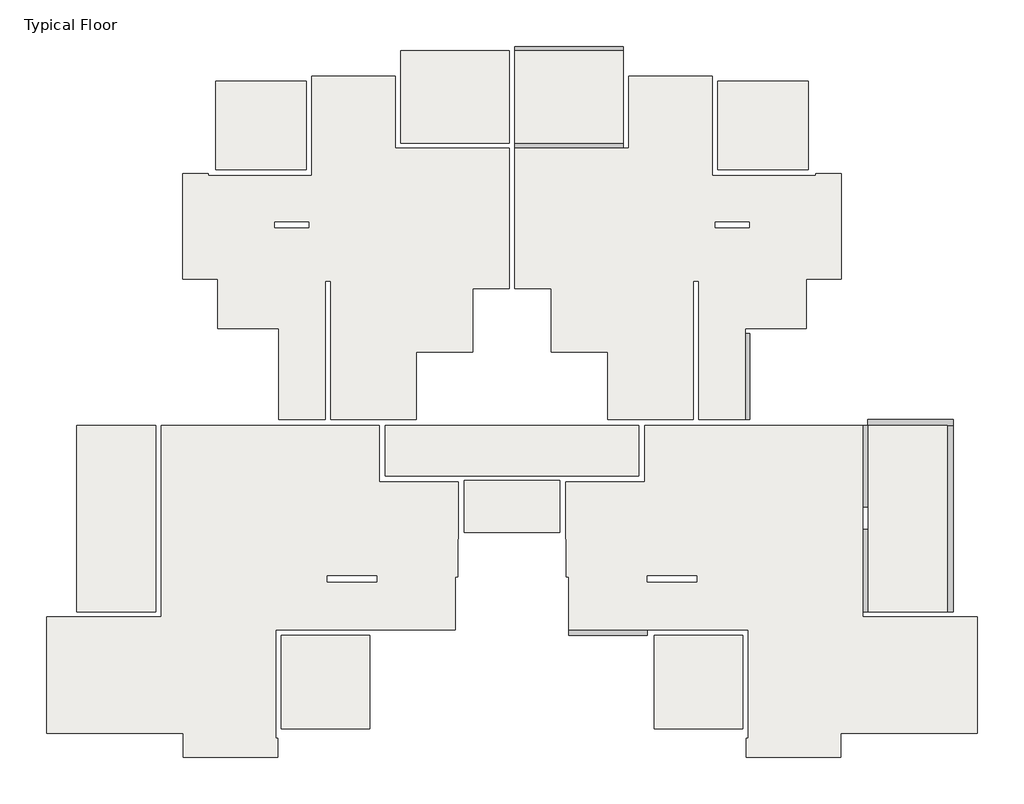
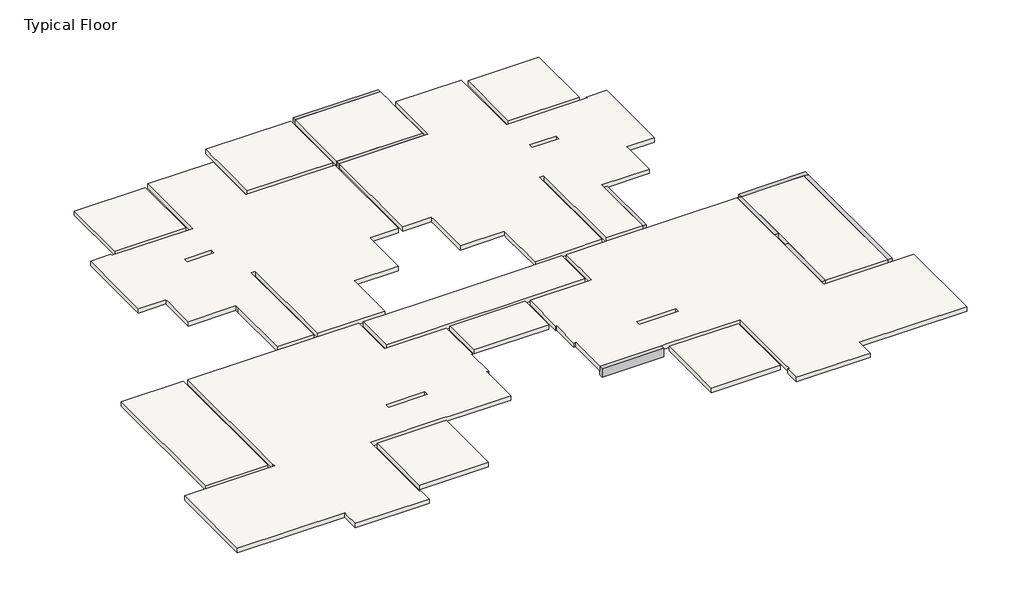
# One storey: 14 slabs, 8 beams.
"""IFC4 building model written with IfcOpenShell, lengths in millimetres."""

from ifc_helpers import new_model, si_unit, frame, origin, place, context, project, spatial, polyline, outline, extrude, faceted_brep, element, save

model = new_model("IFC4")

# Units and contexts
model_context = context("Model", 3, world=origin())
ifc_project = project(units=[si_unit("LENGTHUNIT", "METRE", prefix="MILLI")], contexts=[model_context])

# Site, building, storey
site = spatial("IfcSite", under=ifc_project)
building = spatial("IfcBuilding", under=site)
storey = spatial("IfcBuildingStorey", under=building, Name="Typical Floor", Elevation=2970.0)

# Beams
placement = place(None, origin())
element("IfcBeam", 1, ObjectType="Concrete Rectengular Beam : 15/40", at=placement, inside=storey, context=model_context, shape_type="Brep", body=[
    faceted_brep([(9242.3116422, 3105.4959573, 2970.0), (9092.3116422, 3105.4959573, 2970.0), (9092.3116422, 53.6346435, 2970.0), (9242.3116422, 53.6346435, 2970.0), (9242.3116422, 3105.4959573, 2570.0), (9242.3116422, 53.6346435, 2570.0), (9092.3116422, 3105.4959573, 2570.0), (9092.3116422, 53.6346435, 2570.0), (9092.3116422, 3105.4959573, 2760.0), (9092.3116422, 53.6346435, 2760.0)], [[[0, 1, 2, 3]], [[4, 0, 3, 5]], [[6, 4, 5, 7]], [[2, 1, 8, 6, 7, 9]], [[1, 0, 4, 6, 8]], [[3, 2, 9, 7, 5]]]),
])
element("IfcBeam", 2, ObjectType="Concrete Rectengular Beam : 15/40", at=placement, inside=storey, context=model_context, shape_type="Brep", body=[
    faceted_brep([(4769.8298903, 13127.6127456, 2970.0), (4769.8298903, 13277.6127456, 2970.0), (922.5306203, 13277.6127456, 2970.0), (922.5306203, 13127.6127456, 2970.0), (4769.8298903, 13127.6127456, 2570.0), (4769.8298903, 13127.6127456, 2760.0), (922.5306203, 13127.6127456, 2760.0), (922.5306203, 13127.6127456, 2570.0), (4769.8298903, 13277.6127456, 2570.0), (922.5306203, 13277.6127456, 2570.0)], [[[0, 1, 2, 3]], [[4, 5, 0, 3, 6, 7]], [[8, 4, 7, 9]], [[1, 8, 9, 2]], [[1, 0, 5, 4, 8]], [[3, 2, 9, 7, 6]]]),
])
element("IfcBeam", 3, ObjectType="Concrete Rectengular Beam : 18/40", at=placement, inside=storey, context=model_context, shape_type="Brep", body=[
    faceted_brep([(922.5306203, 9859.0725997, 2970.0), (922.5306203, 9679.0725997, 2970.0), (4769.8298903, 9679.0725997, 2970.0), (4769.8298903, 9859.0725997, 2970.0), (922.5306203, 9679.0725997, 2760.0), (922.5306203, 9679.0725997, 2570.0), (4769.8298903, 9679.0725997, 2570.0), (922.5306203, 9859.0725997, 2570.0), (4769.8298903, 9859.0725997, 2570.0), (922.5306203, 9859.0725997, 2760.0), (4769.8298903, 9859.0725997, 2760.0)], [[[0, 1, 2, 3]], [[1, 4, 5, 6, 2]], [[5, 7, 8, 6]], [[7, 9, 0, 3, 10, 8]], [[1, 0, 9, 7, 5, 4]], [[3, 2, 6, 8, 10]]]),
])
element("IfcBeam", 4, ObjectType="Concrete Rectengular Beam : 20/40", at=placement, inside=storey, context=model_context, shape_type="Brep", body=[
    faceted_brep([(16442.8225911, -146.3653565, 2970.0), (16442.8225911, 53.6346435, 2970.0), (13417.2386495, 53.6346435, 2970.0), (13417.2386495, -146.3653565, 2970.0), (13440.1948538, -146.3653565, 2970.0), (16242.8225911, -146.3653565, 2970.0), (16442.8225911, 53.6346435, 2570.0), (13417.2386495, 53.6346435, 2570.0), (16442.8225911, -146.3653565, 2570.0), (16242.8225911, -146.3653565, 2570.0), (13440.1948538, -146.3653565, 2570.0), (13417.2386495, -146.3653565, 2570.0)], [[[0, 1, 2, 3, 4, 5]], [[1, 6, 7, 2]], [[6, 8, 9, 10, 11, 7]], [[8, 0, 5, 4, 3, 11, 10, 9]], [[3, 2, 7, 11]], [[1, 0, 8, 6]]]),
])
element("IfcBeam", 5, ObjectType="Concrete Rectengular Beam : 20/40", at=placement, inside=storey, context=model_context, shape_type="Brep", body=[
    faceted_brep([(16242.8225911, -6750.8420555, 2970.0), (16442.8225911, -6750.8420555, 2970.0), (16442.8225911, -146.3653565, 2970.0), (16242.8225911, -146.3653565, 2970.0), (16442.8225911, -6750.8420555, 2570.0), (16442.8225911, -146.3653565, 2570.0), (16242.8225911, -6750.8420555, 2570.0), (16242.8225911, -146.3653565, 2570.0), (16242.8225911, -6750.8420555, 2760.0), (16242.8225911, -146.3653565, 2760.0)], [[[0, 1, 2, 3]], [[1, 4, 5, 2]], [[4, 6, 7, 5]], [[6, 8, 0, 3, 9, 7]], [[1, 0, 8, 6, 4]], [[3, 2, 5, 7, 9]]]),
])
element("IfcBeam", 6, ObjectType="Concrete Rectengular Beam : 20/40", at=placement, inside=storey, context=model_context, shape_type="Brep", body=[
    faceted_brep([(13240.1948538, -3042.8252106, 2970.0), (13440.1948538, -3042.8252106, 2970.0), (13440.1948538, -146.3653565, 2970.0), (13417.2386495, -146.3653565, 2970.0), (13240.1948538, -146.3653565, 2970.0), (13440.1948538, -3042.8252106, 2570.0), (13440.1948538, -146.3653565, 2570.0), (13440.1948538, -146.3653565, 2760.0), (13240.1948538, -3042.8252106, 2570.0), (13240.1948538, -146.3653565, 2570.0), (13417.2386495, -146.3653565, 2570.0), (13240.1948538, -146.3653565, 2760.0), (13240.1948538, -3042.8252106, 2760.0)], [[[0, 1, 2, 3, 4]], [[1, 5, 6, 7, 2]], [[5, 8, 9, 10, 6]], [[0, 4, 11, 9, 8, 12]], [[1, 0, 12, 8, 5]], [[2, 7, 6, 10, 9, 11, 4, 3]]]),
])
element("IfcBeam", 7, ObjectType="Concrete Rectengular Beam : 20/40", at=placement, inside=storey, context=model_context, shape_type="Brep", body=[
    faceted_brep([(13440.1948538, -3842.8252106, 2970.0), (13240.1948538, -3842.8252106, 2970.0), (13240.1948538, -6750.8420555, 2970.0), (13440.1948538, -6750.8420555, 2970.0), (13440.1948538, -3842.8252106, 2570.0), (13440.1948538, -6750.8420555, 2760.0), (13440.1948538, -6750.8420555, 2570.0), (13240.1948538, -3842.8252106, 2570.0), (13240.1948538, -6750.8420555, 2570.0), (13240.1948538, -3842.8252106, 2760.0), (13240.1948538, -6750.8420555, 2760.0)], [[[0, 1, 2, 3]], [[4, 0, 3, 5, 6]], [[7, 4, 6, 8]], [[2, 1, 9, 7, 8, 10]], [[1, 0, 4, 7, 9]], [[3, 2, 10, 8, 6, 5]]]),
])
element("IfcBeam", 8, ObjectType="Concrete Rectengular Beam : 20/40", at=placement, inside=storey, context=model_context, shape_type="Brep", body=[
    faceted_brep([(5618.7842881, -7595.8420555, 2970.0), (5618.7842881, -7395.8420555, 2970.0), (2834.5685574, -7395.8420555, 2970.0), (2834.5685574, -7595.8420555, 2970.0), (5618.7842881, -7595.8420555, 2570.0), (2834.5685574, -7595.8420555, 2570.0), (5618.7842881, -7395.8420555, 2570.0), (2834.5685574, -7395.8420555, 2570.0), (5618.7842881, -7395.8420555, 2760.0), (2834.5685574, -7395.8420555, 2760.0)], [[[0, 1, 2, 3]], [[4, 0, 3, 5]], [[6, 4, 5, 7]], [[2, 1, 8, 6, 7, 9]], [[1, 0, 4, 6, 8]], [[3, 2, 9, 7, 5]]]),
])

# Slabs
element("IfcSlab", 9, ObjectType="21", at=placement, inside=storey, context=model_context, shape_type="SweptSolid", body=[
    extrude(outline(polyline([(-4223.7230475, -7595.8420555), (-4223.7230475, -10895.8420555), (-7343.7230475, -10895.8420555), (-7343.7230475, -7595.8420555), (-4223.7230475, -7595.8420555)])), frame((0.0, 0.0, 2760.0), z_axis=(0.0, 0.0, 1.0), x_axis=(1.0, 0.0, 0.0)), (0.0, 0.0, 1.0), 210.0),
])
element("IfcSlab", 10, ObjectType="21", at=placement, inside=storey, context=model_context, shape_type="Brep", body=[
    faceted_brep([(-7473.7230475, -11915.8420555, 2760.0), (-10813.7230475, -11915.8420555, 2760.0), (-10813.7230475, -11250.8420555, 2760.0), (-10813.7230475, -11070.8420555, 2760.0), (-15663.7230475, -11070.8420555, 2760.0), (-15663.7230475, -6930.8420555, 2760.0), (-11593.7230475, -6930.8420555, 2760.0), (-11593.7230475, -6750.8420555, 2760.0), (-11595.1336133, -6750.8420555, 2760.0), (-11595.1336133, -3842.8252106, 2760.0), (-11595.1336133, -3042.8252106, 2760.0), (-11595.1336133, -146.3653565, 2760.0), (-3874.5073169, -146.3653565, 2760.0), (-3874.5073169, -2146.3653565, 2760.0), (-3674.5073169, -2146.3653565, 2760.0), (-1074.5073169, -2146.3653565, 2760.0), (-1074.5073169, -4176.3653565, 2760.0), (-1099.5073169, -4176.3653565, 2760.0), (-1099.5073169, -5521.3653565, 2760.0), (-1189.5073169, -5521.3653565, 2760.0), (-1189.5073169, -7395.8420555, 2760.0), (-3973.7230475, -7395.8420555, 2760.0), (-4223.7230475, -7395.8420555, 2760.0), (-7543.7230475, -7395.8420555, 2760.0), (-7543.7230475, -7595.8420555, 2760.0), (-7543.7230475, -10895.8420555, 2760.0), (-7543.7230475, -11245.8420555, 2760.0), (-7473.7230475, -11245.8420555, 2760.0), (-3974.5402832, -5492.9594837, 2760.0), (-5724.5402832, -5492.9594837, 2760.0), (-5724.5402832, -5692.9594837, 2760.0), (-3974.5402832, -5692.9594837, 2760.0), (-10813.7230475, -11915.8420555, 2970.0), (-10588.7230475, -11915.8420555, 2970.0), (-7703.7230475, -11915.8420555, 2970.0), (-7473.7230475, -11915.8420555, 2970.0), (-7473.7230475, -11245.8420555, 2970.0), (-7543.7230475, -11245.8420555, 2970.0), (-7543.7230475, -10895.8420555, 2970.0), (-7543.7230475, -7595.8420555, 2970.0), (-7543.7230475, -7395.8420555, 2970.0), (-4223.7230475, -7395.8420555, 2970.0), (-3973.7230475, -7395.8420555, 2970.0), (-1189.5073169, -7395.8420555, 2970.0), (-1189.5073169, -5521.3653565, 2970.0), (-1099.5073169, -5521.3653565, 2970.0), (-1099.5073169, -4176.3653565, 2970.0), (-1074.5073169, -4176.3653565, 2970.0), (-1074.5073169, -2146.3653565, 2970.0), (-3674.5073169, -2146.3653565, 2970.0), (-3874.5073169, -2146.3653565, 2970.0), (-3874.5073169, -146.3653565, 2970.0), (-5597.1774089, -146.3653565, 2970.0), (-5797.1774089, -146.3653565, 2970.0), (-11595.1336133, -146.3653565, 2970.0), (-11595.1336133, -3042.8252106, 2970.0), (-11595.1336133, -3842.8252106, 2970.0), (-11595.1336133, -6750.8420555, 2970.0), (-11593.7230475, -6750.8420555, 2970.0), (-11593.7230475, -6930.8420555, 2970.0), (-15663.7230475, -6930.8420555, 2970.0), (-15663.7230475, -11070.8420555, 2970.0), (-10813.7230475, -11070.8420555, 2970.0), (-10813.7230475, -11250.8420555, 2970.0), (-5724.5402832, -5492.9594837, 2970.0), (-3974.5402832, -5492.9594837, 2970.0), (-3974.5402832, -5692.9594837, 2970.0), (-5724.5402832, -5692.9594837, 2970.0)], [[[0, 1, 2, 3, 4, 5, 6, 7, 8, 9, 10, 11, 12, 13, 14, 15, 16, 17, 18, 19, 20, 21, 22, 23, 24, 25, 26, 27], [28, 29, 30, 31]], [[32, 33, 34, 35, 36, 37, 38, 39, 40, 41, 42, 43, 44, 45, 46, 47, 48, 49, 50, 51, 52, 53, 54, 55, 56, 57, 58, 59, 60, 61, 62, 63], [64, 65, 66, 67]], [[1, 0, 35, 34, 33, 32]], [[1, 32, 63, 62, 3, 2]], [[4, 3, 62, 61]], [[5, 4, 61, 60]], [[5, 60, 59, 6]], [[54, 11, 10, 9, 8, 57, 56, 55]], [[12, 11, 54, 53, 52, 51]], [[13, 12, 51, 50]], [[13, 50, 49, 48, 15, 14]], [[16, 15, 48, 47]], [[17, 16, 47, 46]], [[18, 17, 46, 45]], [[19, 18, 45, 44]], [[20, 19, 44, 43]], [[20, 43, 42, 41, 40, 23, 22, 21]], [[23, 40, 39, 38, 37, 26, 25, 24]], [[27, 26, 37, 36]], [[0, 27, 36, 35]], [[29, 28, 65, 64]], [[30, 29, 64, 67]], [[31, 30, 67, 66]], [[28, 31, 66, 65]], [[7, 58, 57, 8]], [[58, 7, 6, 59]]]),
])
element("IfcSlab", 11, ObjectType="21", at=placement, inside=storey, context=model_context, shape_type="Brep", body=[
    faceted_brep([(-14597.7613505, -146.3653565, 2760.0), (-11795.1336133, -146.3653565, 2760.0), (-11795.1336133, -6750.8420555, 2760.0), (-14597.7613505, -6750.8420555, 2760.0), (-11795.1336133, -146.3653565, 2970.0), (-14597.7613505, -146.3653565, 2970.0), (-14597.7613505, -6750.8420555, 2970.0), (-11795.1336133, -6750.8420555, 2970.0), (-11795.1336133, -3842.8252106, 2970.0), (-11795.1336133, -3042.8252106, 2970.0)], [[[0, 1, 2, 3]], [[4, 5, 6, 7, 8, 9]], [[1, 0, 5, 4]], [[2, 1, 4, 9, 8, 7]], [[3, 2, 7, 6]], [[0, 3, 6, 5]]]),
])
element("IfcSlab", 12, ObjectType="21", at=placement, inside=storey, context=model_context, shape_type="SweptSolid", body=[
    extrude(outline(polyline([(-6473.126314, 12055.4959573), (-6473.126314, 8905.4959573), (-9678.126314, 8905.4959573), (-9678.126314, 12055.4959573), (-6473.126314, 12055.4959573)])), frame((0.0, 0.0, 2760.0), z_axis=(0.0, 0.0, 1.0), x_axis=(1.0, 0.0, 0.0)), (0.0, 0.0, 1.0), 210.0),
])
element("IfcSlab", 13, ObjectType="21", at=placement, inside=storey, context=model_context, shape_type="Brep", body=[
    faceted_brep([(722.5306203, 13127.6127456, 2760.0), (722.5306203, 9859.0725997, 2760.0), (-3124.7686498, 9859.0725997, 2760.0), (-3124.7686498, 13127.6127456, 2760.0), (722.5306203, 9859.0725997, 2970.0), (722.5306203, 13127.6127456, 2970.0), (-3124.7686498, 13127.6127456, 2970.0), (-3124.7686498, 12405.4959573, 2970.0), (-3124.7686498, 12225.4959573, 2970.0), (-3124.7686498, 9859.0725997, 2970.0)], [[[0, 1, 2, 3]], [[4, 5, 6, 7, 8, 9]], [[1, 0, 5, 4]], [[1, 4, 9, 2]], [[5, 0, 3, 6]], [[6, 3, 2, 9, 8, 7]]]),
])
element("IfcSlab", 14, ObjectType="21", at=placement, inside=storey, context=model_context, shape_type="Brep", body=[
    faceted_brep([(-6273.126314, 12225.4959573, 2760.0), (-3304.7686498, 12225.4959573, 2760.0), (-3304.7686498, 9679.0725997, 2760.0), (-3124.7686498, 9679.0725997, 2760.0), (722.5306203, 9679.0725997, 2760.0), (722.5306203, 4702.6127456, 2760.0), (-572.4693797, 4702.6127456, 2760.0), (-572.4693797, 4502.6127456, 2760.0), (-572.4693797, 2452.6127456, 2760.0), (-2572.4693797, 2452.6127456, 2760.0), (-2572.4693797, 2252.6127456, 2760.0), (-2572.4693797, 53.6346435, 2760.0), (-5597.1774089, 53.6346435, 2760.0), (-5597.1774089, 4958.6346435, 2760.0), (-5797.1774089, 4958.6346435, 2760.0), (-5797.1774089, 53.6346435, 2760.0), (-7447.2504016, 53.6346435, 2760.0), (-7447.2504016, 3105.4959573, 2760.0), (-7445.6240301, 3105.4959573, 2760.0), (-7445.6240301, 3285.4959573, 2760.0), (-9595.6240301, 3285.4959573, 2760.0), (-9595.6240301, 4855.4959573, 2760.0), (-9595.6240301, 5035.4959573, 2760.0), (-10843.126314, 5035.4959573, 2760.0), (-10843.126314, 8775.4959573, 2760.0), (-9928.126314, 8775.4959573, 2760.0), (-9928.126314, 8705.4959573, 2760.0), (-6473.126314, 8705.4959573, 2760.0), (-6273.126314, 8705.4959573, 2760.0), (-6378.4912775, 7053.4886581, 2760.0), (-7578.4912775, 7053.4886581, 2760.0), (-7578.4912775, 6853.4886581, 2760.0), (-6378.4912775, 6853.4886581, 2760.0), (-3304.7686498, 12225.4959573, 2970.0), (-6273.126314, 12225.4959573, 2970.0), (-6273.126314, 8705.4959573, 2970.0), (-6473.126314, 8705.4959573, 2970.0), (-9928.126314, 8705.4959573, 2970.0), (-9928.126314, 8775.4959573, 2970.0), (-10843.126314, 8775.4959573, 2970.0), (-10843.126314, 5035.4959573, 2970.0), (-9595.6240301, 5035.4959573, 2970.0), (-9595.6240301, 4855.4959573, 2970.0), (-9595.6240301, 3285.4959573, 2970.0), (-7445.6240301, 3285.4959573, 2970.0), (-7445.6240301, 3105.4959573, 2970.0), (-7447.2504016, 3105.4959573, 2970.0), (-7447.2504016, 53.6346435, 2970.0), (-5797.1774089, 53.6346435, 2970.0), (-5797.1774089, 4958.6346435, 2970.0), (-5597.1774089, 4958.6346435, 2970.0), (-5597.1774089, 53.6346435, 2970.0), (-2572.4693797, 53.6346435, 2970.0), (-2572.4693797, 2252.6127456, 2970.0), (-2572.4693797, 2452.6127456, 2970.0), (-572.4693797, 2452.6127456, 2970.0), (-572.4693797, 4502.6127456, 2970.0), (-572.4693797, 4702.6127456, 2970.0), (722.5306203, 4702.6127456, 2970.0), (722.5306203, 9679.0725997, 2970.0), (-3124.7686498, 9679.0725997, 2970.0), (-3304.7686498, 9679.0725997, 2970.0), (-7578.4912775, 7053.4886581, 2970.0), (-6378.4912775, 7053.4886581, 2970.0), (-6378.4912775, 6853.4886581, 2970.0), (-7578.4912775, 6853.4886581, 2970.0)], [[[0, 1, 2, 3, 4, 5, 6, 7, 8, 9, 10, 11, 12, 13, 14, 15, 16, 17, 18, 19, 20, 21, 22, 23, 24, 25, 26, 27, 28], [29, 30, 31, 32]], [[33, 34, 35, 36, 37, 38, 39, 40, 41, 42, 43, 44, 45, 46, 47, 48, 49, 50, 51, 52, 53, 54, 55, 56, 57, 58, 59, 60, 61], [62, 63, 64, 65]], [[1, 0, 34, 33]], [[2, 1, 33, 61]], [[2, 61, 60, 59, 4, 3]], [[5, 4, 59, 58]], [[6, 5, 58, 57]], [[6, 57, 56, 55, 8, 7]], [[9, 8, 55, 54]], [[9, 54, 53, 52, 11, 10]], [[12, 11, 52, 51]], [[13, 12, 51, 50]], [[14, 13, 50, 49]], [[15, 14, 49, 48]], [[16, 15, 48, 47]], [[16, 47, 46, 17]], [[43, 20, 19, 44]], [[20, 43, 42, 41, 22, 21]], [[23, 22, 41, 40]], [[24, 23, 40, 39]], [[25, 24, 39, 38]], [[26, 25, 38, 37]], [[26, 37, 36, 35, 28, 27]], [[0, 28, 35, 34]], [[30, 29, 63, 62]], [[31, 30, 62, 65]], [[32, 31, 65, 64]], [[29, 32, 64, 63]], [[45, 18, 17, 46]], [[18, 45, 44, 19]]]),
])
element("IfcSlab", 15, ObjectType="21", at=placement, inside=storey, context=model_context, shape_type="SweptSolid", body=[
    extrude(outline(polyline([(5868.7842881, -7595.8420555), (8988.7842881, -7595.8420555), (8988.7842881, -10895.8420555), (5868.7842881, -10895.8420555), (5868.7842881, -7595.8420555)])), frame((0.0, 0.0, 2760.0), z_axis=(0.0, 0.0, 1.0), x_axis=(1.0, 0.0, 0.0)), (0.0, 0.0, 1.0), 210.0),
])
element("IfcSlab", 16, ObjectType="21", at=placement, inside=storey, context=model_context, shape_type="Brep", body=[
    faceted_brep([(12458.7842881, -11915.8420555, 2760.0), (9118.7842881, -11915.8420555, 2760.0), (9118.7842881, -11245.8420555, 2760.0), (9188.7842881, -11245.8420555, 2760.0), (9188.7842881, -10895.8420555, 2760.0), (9188.7842881, -7595.8420555, 2760.0), (9188.7842881, -7395.8420555, 2760.0), (5868.7842881, -7395.8420555, 2760.0), (5618.7842881, -7395.8420555, 2760.0), (2834.5685574, -7395.8420555, 2760.0), (2834.5685574, -5521.3653565, 2760.0), (2744.5685574, -5521.3653565, 2760.0), (2744.5685574, -4176.3653565, 2760.0), (2719.5685574, -4176.3653565, 2760.0), (2719.5685574, -2146.3653565, 2760.0), (5319.5685574, -2146.3653565, 2760.0), (5519.5685574, -2146.3653565, 2760.0), (5519.5685574, -146.3653565, 2760.0), (13240.1948538, -146.3653565, 2760.0), (13240.1948538, -3042.8252106, 2760.0), (13240.1948538, -3842.8252106, 2760.0), (13240.1948538, -6750.8420555, 2760.0), (13238.7842881, -6750.8420555, 2760.0), (13238.7842881, -6930.8420555, 2760.0), (17308.7842881, -6930.8420555, 2760.0), (17308.7842881, -11070.8420555, 2760.0), (12458.7842881, -11070.8420555, 2760.0), (12458.7842881, -11250.8420555, 2760.0), (7369.6015237, -5492.9594837, 2760.0), (5619.6015237, -5492.9594837, 2760.0), (5619.6015237, -5692.9594837, 2760.0), (7369.6015237, -5692.9594837, 2760.0), (9118.7842881, -11915.8420555, 2970.0), (9348.7842881, -11915.8420555, 2970.0), (12233.7842881, -11915.8420555, 2970.0), (12458.7842881, -11915.8420555, 2970.0), (12458.7842881, -11250.8420555, 2970.0), (12458.7842881, -11070.8420555, 2970.0), (17308.7842881, -11070.8420555, 2970.0), (17308.7842881, -6930.8420555, 2970.0), (13238.7842881, -6930.8420555, 2970.0), (13238.7842881, -6750.8420555, 2970.0), (13240.1948538, -6750.8420555, 2970.0), (13240.1948538, -3842.8252106, 2970.0), (13240.1948538, -3042.8252106, 2970.0), (13240.1948538, -146.3653565, 2970.0), (7442.2386495, -146.3653565, 2970.0), (7242.2386495, -146.3653565, 2970.0), (5519.5685574, -146.3653565, 2970.0), (5519.5685574, -2146.3653565, 2970.0), (5319.5685574, -2146.3653565, 2970.0), (2719.5685574, -2146.3653565, 2970.0), (2719.5685574, -4176.3653565, 2970.0), (2744.5685574, -4176.3653565, 2970.0), (2744.5685574, -5521.3653565, 2970.0), (2834.5685574, -5521.3653565, 2970.0), (2834.5685574, -7395.8420555, 2970.0), (5618.7842881, -7395.8420555, 2970.0), (5868.7842881, -7395.8420555, 2970.0), (9188.7842881, -7395.8420555, 2970.0), (9188.7842881, -7595.8420555, 2970.0), (9188.7842881, -10895.8420555, 2970.0), (9188.7842881, -11245.8420555, 2970.0), (9118.7842881, -11245.8420555, 2970.0), (5619.6015237, -5492.9594837, 2970.0), (7369.6015237, -5492.9594837, 2970.0), (7369.6015237, -5692.9594837, 2970.0), (5619.6015237, -5692.9594837, 2970.0)], [[[0, 1, 2, 3, 4, 5, 6, 7, 8, 9, 10, 11, 12, 13, 14, 15, 16, 17, 18, 19, 20, 21, 22, 23, 24, 25, 26, 27], [28, 29, 30, 31]], [[32, 33, 34, 35, 36, 37, 38, 39, 40, 41, 42, 43, 44, 45, 46, 47, 48, 49, 50, 51, 52, 53, 54, 55, 56, 57, 58, 59, 60, 61, 62, 63], [64, 65, 66, 67]], [[1, 0, 35, 34, 33, 32]], [[26, 37, 36, 35, 0, 27]], [[26, 25, 38, 37]], [[25, 24, 39, 38]], [[39, 24, 23, 40]], [[18, 45, 44, 43, 42, 21, 20, 19]], [[18, 17, 48, 47, 46, 45]], [[17, 16, 49, 48]], [[14, 51, 50, 49, 16, 15]], [[14, 13, 52, 51]], [[13, 12, 53, 52]], [[12, 11, 54, 53]], [[11, 10, 55, 54]], [[10, 9, 56, 55]], [[6, 59, 58, 57, 56, 9, 8, 7]], [[3, 62, 61, 60, 59, 6, 5, 4]], [[3, 2, 63, 62]], [[2, 1, 32, 63]], [[29, 28, 65, 64]], [[28, 31, 66, 65]], [[31, 30, 67, 66]], [[30, 29, 64, 67]], [[41, 22, 21, 42]], [[40, 23, 22, 41]]]),
])
element("IfcSlab", 17, ObjectType="21", at=placement, inside=storey, context=model_context, shape_type="Brep", body=[
    faceted_brep([(13440.1948538, -146.3653565, 2760.0), (16242.8225911, -146.3653565, 2760.0), (16242.8225911, -6750.8420555, 2760.0), (13440.1948538, -6750.8420555, 2760.0), (16242.8225911, -146.3653565, 2970.0), (13440.1948538, -146.3653565, 2970.0), (13440.1948538, -3042.8252106, 2970.0), (13440.1948538, -3842.8252106, 2970.0), (13440.1948538, -6750.8420555, 2970.0), (16242.8225911, -6750.8420555, 2970.0)], [[[0, 1, 2, 3]], [[4, 5, 6, 7, 8, 9]], [[1, 0, 5, 4]], [[0, 3, 8, 7, 6, 5]], [[3, 2, 9, 8]], [[2, 1, 4, 9]]]),
])
element("IfcSlab", 18, ObjectType="21", at=placement, inside=storey, context=model_context, shape_type="SweptSolid", body=[
    extrude(outline(polyline([(8118.1875546, 12055.4959573), (11323.1875546, 12055.4959573), (11323.1875546, 8905.4959573), (8118.1875546, 8905.4959573), (8118.1875546, 12055.4959573)])), frame((0.0, 0.0, 2760.0), z_axis=(0.0, 0.0, 1.0), x_axis=(1.0, 0.0, 0.0)), (0.0, 0.0, 1.0), 210.0),
])
element("IfcSlab", 19, ObjectType="21", at=placement, inside=storey, context=model_context, shape_type="Brep", body=[
    faceted_brep([(922.5306203, 9859.0725997, 2760.0), (922.5306203, 13127.6127456, 2760.0), (4769.8298903, 13127.6127456, 2760.0), (4769.8298903, 9859.0725997, 2760.0), (922.5306203, 13127.6127456, 2970.0), (922.5306203, 9859.0725997, 2970.0), (4769.8298903, 9859.0725997, 2970.0), (4769.8298903, 12225.4959573, 2970.0), (4769.8298903, 12405.4959573, 2970.0), (4769.8298903, 13127.6127456, 2970.0)], [[[0, 1, 2, 3]], [[4, 5, 6, 7, 8, 9]], [[5, 0, 3, 6]], [[1, 4, 9, 2]], [[1, 0, 5, 4]], [[6, 3, 2, 9, 8, 7]]]),
])
element("IfcSlab", 20, ObjectType="21", at=placement, inside=storey, context=model_context, shape_type="Brep", body=[
    faceted_brep([(4949.8298903, 12225.4959573, 2760.0), (7918.1875546, 12225.4959573, 2760.0), (7918.1875546, 8705.4959573, 2760.0), (8118.1875546, 8705.4959573, 2760.0), (11573.1875546, 8705.4959573, 2760.0), (11573.1875546, 8775.4959573, 2760.0), (12488.1875546, 8775.4959573, 2760.0), (12488.1875546, 5035.4959573, 2760.0), (11240.6852706, 5035.4959573, 2760.0), (11240.6852706, 4855.4959573, 2760.0), (11240.6852706, 3285.4959573, 2760.0), (9090.6852706, 3285.4959573, 2760.0), (9090.6852706, 3105.4959573, 2760.0), (9092.3116422, 3105.4959573, 2760.0), (9092.3116422, 53.6346435, 2760.0), (7442.2386495, 53.6346435, 2760.0), (7442.2386495, 4958.6346435, 2760.0), (7242.2386495, 4958.6346435, 2760.0), (7242.2386495, 53.6346435, 2760.0), (4217.5306203, 53.6346435, 2760.0), (4217.5306203, 2252.6127456, 2760.0), (4217.5306203, 2452.6127456, 2760.0), (2217.5306203, 2452.6127456, 2760.0), (2217.5306203, 4502.6127456, 2760.0), (2217.5306203, 4702.6127456, 2760.0), (922.5306203, 4702.6127456, 2760.0), (922.5306203, 9679.0725997, 2760.0), (4769.8298903, 9679.0725997, 2760.0), (4949.8298903, 9679.0725997, 2760.0), (9223.5525181, 7053.4886581, 2760.0), (8023.5525181, 7053.4886581, 2760.0), (8023.5525181, 6853.4886581, 2760.0), (9223.5525181, 6853.4886581, 2760.0), (7918.1875546, 12225.4959573, 2970.0), (4949.8298903, 12225.4959573, 2970.0), (4949.8298903, 9679.0725997, 2970.0), (4769.8298903, 9679.0725997, 2970.0), (922.5306203, 9679.0725997, 2970.0), (922.5306203, 4702.6127456, 2970.0), (2217.5306203, 4702.6127456, 2970.0), (2217.5306203, 4502.6127456, 2970.0), (2217.5306203, 2452.6127456, 2970.0), (4217.5306203, 2452.6127456, 2970.0), (4217.5306203, 2252.6127456, 2970.0), (4217.5306203, 53.6346435, 2970.0), (7242.2386495, 53.6346435, 2970.0), (7242.2386495, 4958.6346435, 2970.0), (7442.2386495, 4958.6346435, 2970.0), (7442.2386495, 53.6346435, 2970.0), (9092.3116422, 53.6346435, 2970.0), (9092.3116422, 3105.4959573, 2970.0), (9090.6852706, 3105.4959573, 2970.0), (9090.6852706, 3285.4959573, 2970.0), (11240.6852706, 3285.4959573, 2970.0), (11240.6852706, 4855.4959573, 2970.0), (11240.6852706, 5035.4959573, 2970.0), (12488.1875546, 5035.4959573, 2970.0), (12488.1875546, 8775.4959573, 2970.0), (11573.1875546, 8775.4959573, 2970.0), (11573.1875546, 8705.4959573, 2970.0), (8118.1875546, 8705.4959573, 2970.0), (7918.1875546, 8705.4959573, 2970.0), (8023.5525181, 7053.4886581, 2970.0), (9223.5525181, 7053.4886581, 2970.0), (9223.5525181, 6853.4886581, 2970.0), (8023.5525181, 6853.4886581, 2970.0)], [[[0, 1, 2, 3, 4, 5, 6, 7, 8, 9, 10, 11, 12, 13, 14, 15, 16, 17, 18, 19, 20, 21, 22, 23, 24, 25, 26, 27, 28], [29, 30, 31, 32]], [[33, 34, 35, 36, 37, 38, 39, 40, 41, 42, 43, 44, 45, 46, 47, 48, 49, 50, 51, 52, 53, 54, 55, 56, 57, 58, 59, 60, 61], [62, 63, 64, 65]], [[1, 0, 34, 33]], [[0, 28, 35, 34]], [[35, 28, 27, 26, 37, 36]], [[24, 39, 38, 25]], [[22, 41, 40, 39, 24, 23]], [[22, 21, 42, 41]], [[19, 44, 43, 42, 21, 20]], [[19, 18, 45, 44]], [[18, 17, 46, 45]], [[17, 16, 47, 46]], [[16, 15, 48, 47]], [[15, 14, 49, 48]], [[49, 14, 13, 50]], [[10, 53, 52, 11]], [[8, 55, 54, 53, 10, 9]], [[8, 7, 56, 55]], [[7, 6, 57, 56]], [[6, 5, 58, 57]], [[5, 4, 59, 58]], [[2, 61, 60, 59, 4, 3]], [[2, 1, 33, 61]], [[30, 29, 63, 62]], [[29, 32, 64, 63]], [[32, 31, 65, 64]], [[31, 30, 62, 65]], [[12, 51, 50, 13]], [[11, 52, 51, 12]], [[26, 25, 38, 37]]]),
])
element("IfcSlab", 21, ObjectType="21", at=placement, inside=storey, context=model_context, shape_type="Brep", body=[
    faceted_brep([(2519.5685574, -3946.3653565, 2760.0), (-874.5073169, -3946.3653565, 2760.0), (-874.5073169, -2096.3653565, 2760.0), (2519.5685574, -2096.3653565, 2760.0), (2519.5685574, -3946.3653565, 2970.0), (2519.5685574, -2146.3653565, 2970.0), (2519.5685574, -2096.3653565, 2970.0), (-874.5073169, -2096.3653565, 2970.0), (-874.5073169, -2146.3653565, 2970.0), (-874.5073169, -3946.3653565, 2970.0)], [[[0, 1, 2, 3]], [[4, 5, 6, 7, 8, 9]], [[1, 0, 4, 9]], [[2, 1, 9, 8, 7]], [[3, 2, 7, 6]], [[0, 3, 6, 5, 4]]]),
])
element("IfcSlab", 22, ObjectType="21", at=placement, inside=storey, context=model_context, shape_type="Brep", body=[
    faceted_brep([(5319.5685574, -146.3653565, 2760.0), (5319.5685574, -1946.3653565, 2760.0), (-3674.5073169, -1946.3653565, 2760.0), (-3674.5073169, -146.3653565, 2760.0), (5319.5685574, -1946.3653565, 2970.0), (5319.5685574, -146.3653565, 2970.0), (2622.2386495, -146.3653565, 2970.0), (2217.5306203, -146.3653565, 2970.0), (2017.5306203, -146.3653565, 2970.0), (-372.4693797, -146.3653565, 2970.0), (-572.4693797, -146.3653565, 2970.0), (-977.1774089, -146.3653565, 2970.0), (-3674.5073169, -146.3653565, 2970.0), (-3674.5073169, -1946.3653565, 2970.0), (-874.5073169, -1946.3653565, 2970.0), (2519.5685574, -1946.3653565, 2970.0)], [[[0, 1, 2, 3]], [[4, 5, 6, 7, 8, 9, 10, 11, 12, 13, 14, 15]], [[1, 0, 5, 4]], [[2, 1, 4, 15, 14, 13]], [[3, 2, 13, 12]], [[0, 3, 12, 11, 10, 9, 8, 7, 6, 5]]]),
])

save(model, "model.ifc")

# Revit data of these elements
# Type "Concrete Rectengular Beam : 15/40"
#   Length [instance default] = 152.4 cm
#   b = 15 cm
#   h = 40 cm
#   Structural Material [instance default] = Concrete
#   Assembly Code = ""
# Type "Concrete Rectengular Beam : 18/40"
#   Length [instance default] = 152.4 cm
#   b = 18 cm
#   h = 40 cm
#   Structural Material [instance default] = Concrete
#   Assembly Code = ""
# Type "Concrete Rectengular Beam : 20/40"
#   Keynote = "09000"
#   Length [instance default] = 152.4 cm
#   b = 20 cm
#   h = 40 cm
#   Structural Material [instance default] = Concrete
#   Assembly Code = ""
# Type "21"
#   Function = 0
#   Layers, outside or top first: 21 cm "Concrete" (function 1)
# Element 1 (IfcBeam, "Concrete Rectengular Beam : 15/40")
#   Comments = ""
#   Mark = "B3"
#   SOFiSTiK_AMG_Comments = ""
#   SOFiSTiK_AMG_Scheduled = yes
#   SOFiSTiK_AMG_Adjusted = yes
#   Structural Material = Concrete
#   Phase Created = New Construction
#   Materials on its faces: "Concrete"
# Element 2 (IfcBeam, "Concrete Rectengular Beam : 15/40")
#   Comments = ""
#   Mark = "B4"
#   SOFiSTiK_AMG_Comments = ""
#   SOFiSTiK_AMG_Scheduled = yes
#   SOFiSTiK_AMG_Adjusted = yes
#   Structural Material = Concrete
#   Phase Created = New Construction
#   Materials on its faces: "Concrete"
# Element 3 (IfcBeam, "Concrete Rectengular Beam : 18/40")
#   Comments = ""
#   Mark = "B7"
#   SOFiSTiK_AMG_Comments = ""
#   SOFiSTiK_AMG_Scheduled = yes
#   SOFiSTiK_AMG_Adjusted = yes
#   Structural Material = Concrete
#   Phase Created = New Construction
#   Materials on its faces: "Concrete"
# Element 4 (IfcBeam, "Concrete Rectengular Beam : 20/40")
#   Comments = ""
#   Mark = "B13"
#   SOFiSTiK_AMG_Comments = ""
#   SOFiSTiK_AMG_Scheduled = yes
#   SOFiSTiK_AMG_Adjusted = yes
#   Structural Material = Concrete
#   Phase Created = New Construction
#   Materials on its faces: "Concrete"
# Element 5 (IfcBeam, "Concrete Rectengular Beam : 20/40")
#   Comments = ""
#   Mark = "B14"
#   SOFiSTiK_AMG_Comments = ""
#   SOFiSTiK_AMG_Scheduled = yes
#   SOFiSTiK_AMG_Adjusted = yes
#   Structural Material = Concrete
#   Phase Created = New Construction
#   Materials on its faces: "Concrete"
# Element 6 (IfcBeam, "Concrete Rectengular Beam : 20/40")
#   Comments = ""
#   Mark = "B15"
#   SOFiSTiK_AMG_Comments = ""
#   SOFiSTiK_AMG_Scheduled = yes
#   SOFiSTiK_AMG_Adjusted = yes
#   Structural Material = Concrete
#   Phase Created = New Construction
#   Materials on its faces: "Concrete"
# Element 7 (IfcBeam, "Concrete Rectengular Beam : 20/40")
#   Comments = ""
#   Mark = "B16"
#   SOFiSTiK_AMG_Comments = ""
#   SOFiSTiK_AMG_Scheduled = yes
#   SOFiSTiK_AMG_Adjusted = yes
#   Structural Material = Concrete
#   Phase Created = New Construction
#   Materials on its faces: "Concrete"
# Element 8 (IfcBeam, "Concrete Rectengular Beam : 20/40")
#   Comments = ""
#   Mark = "B17"
#   SOFiSTiK_AMG_Comments = ""
#   SOFiSTiK_AMG_Scheduled = yes
#   SOFiSTiK_AMG_Adjusted = yes
#   Structural Material = Concrete
#   Phase Created = New Construction
#   Materials on its faces: "Concrete"
# Element 9 (IfcSlab, "21")
#   Mark = "S1"
#   SOFiSTiK_AMG_Comments = ""
#   Height Offset From Level = 0 cm
#   built-in parameter 1001954 = 1
#   SOFiSTiK_AMG_Scheduled = yes
#   SOFiSTiK_AMG_Adjusted = yes
#   Phase Created = New Construction
#   Materials on its faces: "Concrete"
# Element 10 (IfcSlab, "21")
#   Mark = "S2"
#   SOFiSTiK_AMG_Comments = ""
#   Height Offset From Level = 0 cm
#   built-in parameter 1001954 = 1
#   SOFiSTiK_AMG_Scheduled = yes
#   SOFiSTiK_AMG_Adjusted = yes
#   Phase Created = New Construction
#   Materials on its faces: "Concrete"
# Element 11 (IfcSlab, "21")
#   Mark = "S3"
#   SOFiSTiK_AMG_Comments = ""
#   built-in parameter 1001955 = 3.14159 (stored number, unit not read)
#   Height Offset From Level = 0 cm
#   built-in parameter 1001954 = 1
#   SOFiSTiK_AMG_Scheduled = yes
#   SOFiSTiK_AMG_Adjusted = yes
#   Phase Created = New Construction
#   Materials on its faces: "Concrete"
# Element 12 (IfcSlab, "21")
#   Mark = "S4"
#   SOFiSTiK_AMG_Comments = ""
#   Height Offset From Level = 0 cm
#   built-in parameter 1001954 = 1
#   SOFiSTiK_AMG_Scheduled = yes
#   SOFiSTiK_AMG_Adjusted = yes
#   Phase Created = New Construction
#   Materials on its faces: "Concrete"
# Element 13 (IfcSlab, "21")
#   Mark = "S5"
#   SOFiSTiK_AMG_Comments = ""
#   Height Offset From Level = 0 cm
#   built-in parameter 1001954 = 1
#   SOFiSTiK_AMG_Scheduled = yes
#   SOFiSTiK_AMG_Adjusted = yes
#   Phase Created = New Construction
#   Materials on its faces: "Concrete"
# Element 14 (IfcSlab, "21")
#   Mark = "S6"
#   SOFiSTiK_AMG_Comments = ""
#   built-in parameter 1001955 = 3.14159 (stored number, unit not read)
#   Height Offset From Level = 0 cm
#   built-in parameter 1001954 = 1
#   SOFiSTiK_AMG_Scheduled = yes
#   SOFiSTiK_AMG_Adjusted = yes
#   Phase Created = New Construction
#   Materials on its faces: "Concrete"
# Element 15 (IfcSlab, "21")
#   Mark = "S7"
#   SOFiSTiK_AMG_Comments = ""
#   built-in parameter 1001955 = 3.14159 (stored number, unit not read)
#   Height Offset From Level = 0 cm
#   built-in parameter 1001954 = 1
#   SOFiSTiK_AMG_Scheduled = yes
#   SOFiSTiK_AMG_Adjusted = yes
#   Phase Created = New Construction
#   Materials on its faces: "Concrete"
# Element 16 (IfcSlab, "21")
#   Mark = "S8"
#   SOFiSTiK_AMG_Comments = ""
#   built-in parameter 1001955 = 3.14159 (stored number, unit not read)
#   Height Offset From Level = 0 cm
#   built-in parameter 1001954 = 1
#   SOFiSTiK_AMG_Scheduled = yes
#   SOFiSTiK_AMG_Adjusted = yes
#   Phase Created = New Construction
#   Materials on its faces: "Concrete"
# Element 17 (IfcSlab, "21")
#   Mark = "S9"
#   SOFiSTiK_AMG_Comments = ""
#   built-in parameter 1001955 = 0 (stored number, unit not read)
#   Height Offset From Level = 0 cm
#   built-in parameter 1001954 = 1
#   SOFiSTiK_AMG_Scheduled = yes
#   SOFiSTiK_AMG_Adjusted = yes
#   Phase Created = New Construction
#   Materials on its faces: "Concrete"
# Element 18 (IfcSlab, "21")
#   Mark = "S10"
#   SOFiSTiK_AMG_Comments = ""
#   built-in parameter 1001955 = 3.14159 (stored number, unit not read)
#   Height Offset From Level = 0 cm
#   built-in parameter 1001954 = 1
#   SOFiSTiK_AMG_Scheduled = yes
#   SOFiSTiK_AMG_Adjusted = yes
#   Phase Created = New Construction
#   Materials on its faces: "Concrete"
# Element 19 (IfcSlab, "21")
#   Mark = "S11"
#   SOFiSTiK_AMG_Comments = ""
#   built-in parameter 1001955 = 3.14159 (stored number, unit not read)
#   Height Offset From Level = 0 cm
#   built-in parameter 1001954 = 1
#   SOFiSTiK_AMG_Scheduled = yes
#   SOFiSTiK_AMG_Adjusted = yes
#   Phase Created = New Construction
#   Materials on its faces: "Concrete"
# Element 20 (IfcSlab, "21")
#   Mark = "S12"
#   SOFiSTiK_AMG_Comments = ""
#   built-in parameter 1001955 = 0 (stored number, unit not read)
#   Height Offset From Level = 0 cm
#   built-in parameter 1001954 = 1
#   SOFiSTiK_AMG_Scheduled = yes
#   SOFiSTiK_AMG_Adjusted = yes
#   Phase Created = New Construction
#   Materials on its faces: "Concrete"
# Element 21 (IfcSlab, "21")
#   Mark = "S13"
#   SOFiSTiK_AMG_Comments = ""
#   Height Offset From Level = 0 cm
#   built-in parameter 1001954 = 1
#   SOFiSTiK_AMG_Scheduled = yes
#   SOFiSTiK_AMG_Adjusted = yes
#   Phase Created = New Construction
#   Materials on its faces: "Concrete"
# Element 22 (IfcSlab, "21")
#   Mark = "S14"
#   SOFiSTiK_AMG_Comments = ""
#   Height Offset From Level = 0 cm
#   built-in parameter 1001954 = 1
#   SOFiSTiK_AMG_Scheduled = yes
#   SOFiSTiK_AMG_Adjusted = yes
#   Phase Created = New Construction
#   Materials on its faces: "Concrete"
# Materials
#   "Concrete": class "Concrete", colour RGB 192 192 192, transparency 0, Keynote = "01000", Description = "Cast-in-place concrete", Cost = 0
